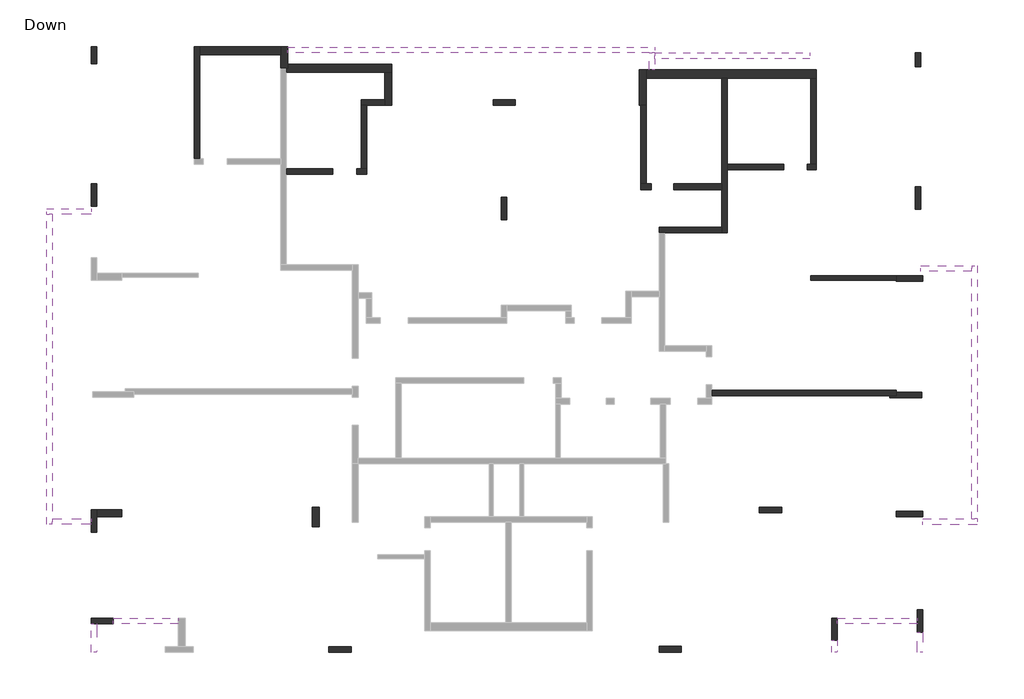
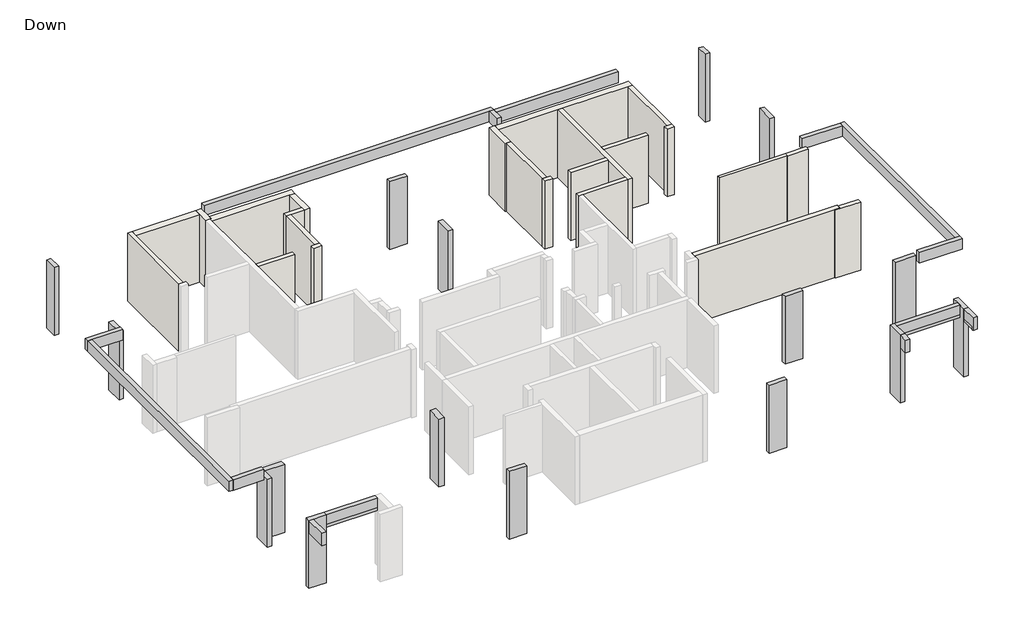
# One storey, part 2 of 2: 23 walls, 16 columns, 14 beams.
"""IFC4 building model written with IfcOpenShell, lengths in millimetres."""

from ifc_helpers import new_model, si_unit, origin, place, context, project, spatial, faceted_brep, element, save

model = new_model("IFC4")

# Units and contexts
model_context = context("Model", 3, world=origin())
ifc_project = project(units=[si_unit("LENGTHUNIT", "METRE", prefix="MILLI")], contexts=[model_context])

# Site, building, storey
site = spatial("IfcSite", under=ifc_project)
building = spatial("IfcBuilding", under=site)
storey = spatial("IfcBuildingStorey", under=building, Name="Down", Elevation=0.0)

# Beams
placement = place(None, origin())
element("IfcBeam", 1, ObjectType="Concrete Rectengular Beam : 20/50", at=placement, inside=storey, context=model_context, shape_type="Brep", body=[
    faceted_brep([(-24231.4241546, 32724.6697375, 3070.0), (-24231.4241546, 32924.6697375, 3070.0), (-24231.4241546, 32924.6697375, 3270.0), (-24231.4241546, 32924.6697375, 3570.0), (-24231.4241546, 32724.6697375, 3570.0), (-24231.4241546, 32724.6697375, 3270.0), (-25831.5472348, 32924.6697375, 3570.0), (-25831.5472348, 32724.6697375, 3570.0), (-25631.5472348, 32724.6697375, 3570.0), (-25831.5472348, 32924.6697375, 3070.0), (-25631.5472348, 32724.6697375, 3070.0), (-25831.5472348, 32724.6697375, 3070.0)], [[[0, 1, 2, 3, 4, 5]], [[4, 3, 6, 7, 8]], [[6, 3, 2, 1, 9]], [[1, 0, 10, 11, 9]], [[4, 8, 7, 11, 10, 0, 5]], [[7, 6, 9, 11]]]),
])
element("IfcBeam", 2, ObjectType="Concrete Rectengular Beam : 20/50", at=placement, inside=storey, context=model_context, shape_type="Brep", body=[
    faceted_brep([(-25831.5472348, 21596.8353122, 3570.0), (-25631.5472348, 21596.8353122, 3570.0), (-25631.5472348, 21796.8353122, 3570.0), (-25631.5472348, 32724.6697375, 3570.0), (-25831.5472348, 32724.6697375, 3570.0), (-25831.5472348, 21596.8353122, 3070.0), (-25831.5472348, 32724.6697375, 3070.0), (-25631.5472348, 21596.8353122, 3070.0), (-25631.5472348, 32724.6697375, 3070.0), (-25631.5472348, 26152.7259194, 3070.0), (-25631.5472348, 21796.8353122, 3070.0), (-25631.5472348, 32724.6697375, 3270.0)], [[[0, 1, 2, 3, 4]], [[5, 0, 4, 6]], [[7, 5, 6, 8, 9, 10]], [[1, 7, 10, 9, 8, 11, 3, 2]], [[1, 0, 5, 7]], [[4, 3, 11, 8, 6]]]),
])
element("IfcBeam", 3, ObjectType="Concrete Rectengular Beam : 20/50", at=placement, inside=storey, context=model_context, shape_type="Brep", body=[
    faceted_brep([(-24232.496199, 21796.8353122, 3570.0), (-24232.496199, 21596.8353122, 3570.0), (-24232.496199, 21596.8353122, 3070.0), (-24232.496199, 21796.8353122, 3070.0), (-24232.496199, 21796.8353122, 3270.0), (-25631.5472348, 21796.8353122, 3570.0), (-25631.5472348, 21596.8353122, 3570.0), (-25631.5472348, 21596.8353122, 3070.0), (-25631.5472348, 21796.8353122, 3070.0), (-25631.5472348, 21796.8353122, 3270.0)], [[[0, 1, 2, 3, 4]], [[1, 0, 5, 6]], [[2, 1, 6, 7]], [[3, 2, 7, 8]], [[4, 3, 8, 9, 5, 0]], [[6, 5, 9, 8, 7]]]),
])
element("IfcBeam", 4, ObjectType="Concrete Rectengular Beam : 20/50", at=placement, inside=storey, context=model_context, shape_type="Brep", body=[
    faceted_brep([(5620.732608, 21792.2762684, 3070.0), (5620.732608, 21592.2762684, 3070.0), (5620.732608, 21592.2762684, 3270.0), (5620.732608, 21592.2762684, 3570.0), (5620.732608, 21792.2762684, 3570.0), (5620.732608, 21792.2762684, 3270.0), (7576.2745907, 21592.2762684, 3570.0), (7576.2745907, 21792.2762684, 3570.0), (7376.2745907, 21792.2762684, 3570.0), (7576.2745907, 21592.2762684, 3070.0), (7376.2745907, 21792.2762684, 3070.0), (7576.2745907, 21792.2762684, 3070.0)], [[[0, 1, 2, 3, 4, 5]], [[4, 3, 6, 7, 8]], [[6, 3, 2, 1, 9]], [[1, 0, 10, 11, 9]], [[4, 8, 7, 11, 10, 0, 5]], [[7, 6, 9, 11]]]),
])
element("IfcBeam", 5, ObjectType="Concrete Rectengular Beam : 20/50", at=placement, inside=storey, context=model_context, shape_type="Brep", body=[
    faceted_brep([(7576.2745907, 30886.4079799, 3570.0), (7376.2745907, 30886.4079799, 3570.0), (7376.2745907, 30686.4079799, 3570.0), (7376.2745907, 21792.2762684, 3570.0), (7576.2745907, 21792.2762684, 3570.0), (7576.2745907, 30886.4079799, 3070.0), (7576.2745907, 21792.2762684, 3070.0), (7376.2745907, 30886.4079799, 3070.0), (7376.2745907, 21792.2762684, 3070.0), (7376.2745907, 26346.3859634, 3070.0), (7376.2745907, 30686.4079799, 3070.0), (7376.2745907, 21792.2762684, 3270.0)], [[[0, 1, 2, 3, 4]], [[5, 0, 4, 6]], [[7, 5, 6, 8, 9, 10]], [[1, 7, 10, 9, 8, 11, 3, 2]], [[4, 3, 11, 8, 6]], [[1, 0, 5, 7]]]),
])
element("IfcBeam", 6, ObjectType="Concrete Rectengular Beam : 20/50", at=placement, inside=storey, context=model_context, shape_type="Brep", body=[
    faceted_brep([(5547.5722379, 30686.4079799, 3570.0), (5547.5722379, 30886.4079799, 3570.0), (5547.5722379, 30886.4079799, 3070.0), (5547.5722379, 30686.4079799, 3070.0), (5547.5722379, 30686.4079799, 3270.0), (7376.2745907, 30686.4079799, 3570.0), (7376.2745907, 30886.4079799, 3570.0), (7376.2745907, 30886.4079799, 3070.0), (7376.2745907, 30686.4079799, 3070.0), (7376.2745907, 30686.4079799, 3270.0)], [[[0, 1, 2, 3, 4]], [[1, 0, 5, 6]], [[2, 1, 6, 7]], [[3, 2, 7, 8]], [[3, 8, 9, 5, 0, 4]], [[7, 6, 5, 9, 8]]]),
])
element("IfcBeam", 7, ObjectType="Concrete Rectengular Beam : 20/50", at=placement, inside=storey, context=model_context, shape_type="Brep", body=[
    faceted_brep([(-17181.9731082, 38714.5374263, 3570.0), (-17181.9731082, 38714.5374263, 3070.0), (-17181.9731082, 38514.5374263, 3070.0), (-17181.9731082, 38514.5374263, 3270.0), (-17181.9731082, 38514.5374263, 3570.0), (-4202.3443382, 38514.5374263, 3570.0), (-4002.3443382, 38514.5374263, 3570.0), (-4002.3443382, 38515.575292, 3570.0), (-4002.3443382, 38714.5374263, 3570.0), (-13700.7193614, 38514.5374263, 3070.0), (-4202.3443382, 38514.5374263, 3070.0), (-4002.3443382, 38514.5374263, 3070.0), (-4002.3443382, 38714.5374263, 3070.0), (-4002.3443382, 38515.575292, 3070.0)], [[[0, 1, 2, 3, 4]], [[0, 4, 5, 6, 7, 8]], [[4, 3, 2, 9, 10, 11, 6, 5]], [[2, 1, 12, 13, 11, 10, 9]], [[1, 0, 8, 12]], [[8, 7, 6, 11, 13, 12]]]),
])
element("IfcBeam", 8, ObjectType="Concrete Rectengular Beam : 20/52", at=placement, inside=storey, context=model_context, shape_type="Brep", body=[
    faceted_brep([(-4002.3443382, 37914.469069, 3570.0), (-4202.3443382, 37914.469069, 3570.0), (-4202.3443382, 37914.469069, 3270.0), (-4202.3443382, 37914.469069, 3070.0), (-4202.3443382, 37914.469069, 3050.0), (-4002.3443382, 37914.469069, 3050.0), (-4002.3443382, 37914.469069, 3070.0), (-4002.3443382, 37914.469069, 3220.0), (-4002.3443382, 38315.575292, 3570.0), (-4002.3443382, 38514.5374263, 3570.0), (-4202.3443382, 38514.5374263, 3570.0), (-4202.3443382, 38515.575292, 3050.0), (-4202.3443382, 38514.5374263, 3270.0), (-4202.3443382, 38514.5374263, 3070.0), (-4202.3443382, 38515.575292, 3070.0), (-4002.3443382, 38515.575292, 3050.0), (-4002.3443382, 38315.575292, 3050.0), (-4002.3443382, 38515.575292, 3070.0), (-4002.3443382, 38514.5374263, 3070.0)], [[[0, 1, 2, 3, 4, 5, 6, 7]], [[1, 0, 8, 9, 10]], [[11, 4, 3, 2, 1, 10, 12, 13, 14]], [[5, 4, 11, 15, 16]], [[0, 7, 6, 5, 16, 15, 17, 18, 9, 8]], [[15, 11, 14, 17]], [[18, 13, 12, 10, 9]], [[13, 18, 17, 14]]]),
])
element("IfcBeam", 9, ObjectType="Concrete Rectengular Beam : 20/52", at=placement, inside=storey, context=model_context, shape_type="Brep", body=[
    faceted_brep([(1566.3525769, 38515.575292, 3570.0), (1566.3525769, 38315.575292, 3570.0), (1566.3525769, 38315.575292, 3270.0), (1566.3525769, 38315.575292, 3070.0), (1566.3525769, 38315.575292, 3050.0), (1566.3525769, 38515.575292, 3050.0), (1566.3525769, 38515.575292, 3070.0), (1566.3525769, 38515.575292, 3270.0), (-4002.3443382, 38515.575292, 3570.0), (-4002.3443382, 38514.5374263, 3570.0), (-4002.3443382, 38315.575292, 3570.0), (-4002.3443382, 38315.575292, 3050.0), (-4002.3443382, 38515.575292, 3050.0), (-4002.3443382, 38515.575292, 3070.0)], [[[0, 1, 2, 3, 4, 5, 6, 7]], [[1, 0, 8, 9, 10]], [[11, 4, 3, 2, 1, 10]], [[5, 4, 11, 12]], [[5, 12, 13, 8, 0, 7, 6]], [[11, 10, 9, 8, 13, 12]]]),
])
element("IfcBeam", 10, ObjectType="Concrete Rectengular Beam : 20/60", at=placement, inside=storey, context=model_context, shape_type="Brep", body=[
    faceted_brep([(5420.732608, 18035.7075634, 3270.0), (5420.732608, 18235.7075634, 3270.0), (2546.318889, 18235.7075634, 3270.0), (2546.318889, 18035.7075634, 3270.0), (2546.318889, 18235.7075634, 2670.0), (2546.318889, 18235.7075634, 3070.0), (5420.732608, 18235.7075634, 3070.0), (5420.732608, 18235.7075634, 2670.0), (5420.732608, 18040.7075634, 2670.0), (2546.318889, 18040.7075634, 2670.0), (2546.318889, 18035.7075634, 2820.0), (5420.732608, 18035.7075634, 2820.0), (5420.732608, 18040.7075634, 2820.0), (2546.318889, 18040.7075634, 2820.0)], [[[0, 1, 2, 3]], [[4, 5, 2, 1, 6, 7]], [[4, 7, 8, 9]], [[0, 3, 10, 11]], [[1, 0, 11, 12, 8, 7, 6]], [[3, 2, 5, 4, 9, 13, 10]], [[13, 12, 11, 10]], [[12, 13, 9, 8]]]),
])
element("IfcBeam", 11, ObjectType="Concrete Rectengular Beam : 20/60", at=placement, inside=storey, context=model_context, shape_type="Brep", body=[
    faceted_brep([(2546.318889, 17016.7180677, 3270.0), (2346.318889, 17016.7180677, 3270.0), (2346.318889, 17016.7180677, 3070.0), (2346.318889, 17016.7180677, 2670.0), (2546.318889, 17016.7180677, 2670.0), (2546.318889, 17435.7075634, 3270.0), (2346.318889, 17435.7075634, 3270.0), (2346.318889, 17435.7075634, 3070.0), (2346.318889, 17435.7075634, 2670.0), (2541.318889, 17435.7075634, 2670.0), (2541.318889, 17066.3078446, 2670.0), (2546.318889, 17066.3078446, 2670.0), (2546.318889, 17066.3078446, 2820.0), (2546.318889, 17435.7075634, 2820.0), (2541.318889, 17435.7075634, 2820.0), (2541.318889, 17066.3078446, 2820.0)], [[[0, 1, 2, 3, 4]], [[1, 0, 5, 6]], [[1, 6, 7, 8, 3, 2]], [[4, 3, 8, 9, 10, 11]], [[0, 4, 11, 12, 13, 5]], [[6, 5, 13, 14, 9, 8, 7]], [[12, 15, 14, 13]], [[10, 15, 12, 11]], [[15, 10, 9, 14]]]),
])
element("IfcBeam", 12, ObjectType="Concrete Rectengular Beam : 20/60", at=placement, inside=storey, context=model_context, shape_type="Brep", body=[
    faceted_brep([(5620.732608, 17010.2006534, 3270.0), (5420.732608, 17010.2006534, 3270.0), (5420.732608, 17010.2006534, 2670.0), (5620.732608, 17010.2006534, 2670.0), (5620.732608, 17735.2006534, 3270.0), (5420.732608, 17735.2006534, 3270.0), (5420.732608, 17735.2006534, 2820.0), (5420.732608, 17066.3078446, 2820.0), (5420.732608, 17066.3078446, 2670.0), (5430.732608, 17066.3078446, 2670.0), (5430.732608, 17735.2006534, 2670.0), (5620.732608, 17735.2006534, 2670.0), (5430.732608, 17735.2006534, 2820.0), (5430.732608, 17066.3078446, 2820.0)], [[[0, 1, 2, 3]], [[1, 0, 4, 5]], [[2, 1, 5, 6, 7, 8]], [[3, 2, 8, 9, 10, 11]], [[0, 3, 11, 4]], [[5, 4, 11, 10, 12, 6]], [[13, 7, 6, 12]], [[13, 9, 8, 7]], [[9, 13, 12, 10]]]),
])
element("IfcBeam", 13, ObjectType="Concrete Rectengular Beam : 20/60", at=placement, inside=storey, context=model_context, shape_type="Brep", body=[
    faceted_brep([(-23432.496199, 18236.7796078, 3270.0), (-23432.496199, 18036.7796078, 3270.0), (-21102.3452666, 18036.7796078, 3270.0), (-21102.3452666, 18236.7796078, 3270.0), (-23432.496199, 18036.7796078, 2820.0), (-21102.3452666, 18036.7796078, 2820.0), (-23432.496199, 18236.7796078, 2670.0), (-21102.3452666, 18236.7796078, 2670.0), (-21102.3452666, 18038.5478478, 2670.0), (-23432.496199, 18038.5478478, 2670.0), (-21102.3452666, 18236.7796078, 3070.0), (-23432.496199, 18236.7796078, 3070.0), (-23432.496199, 18038.5478478, 2820.0), (-21102.3452666, 18038.5478478, 2820.0)], [[[0, 1, 2, 3]], [[2, 1, 4, 5]], [[6, 7, 8, 9]], [[3, 10, 7, 6, 11, 0]], [[1, 0, 11, 6, 9, 12, 4]], [[3, 2, 5, 13, 8, 7, 10]], [[12, 13, 5, 4]], [[13, 12, 9, 8]]]),
])
element("IfcBeam", 14, ObjectType="Concrete Rectengular Beam : 20/60", at=placement, inside=storey, context=model_context, shape_type="Brep", body=[
    faceted_brep([(-24032.496199, 17016.7796078, 3270.0), (-24232.496199, 17016.7796078, 3270.0), (-24232.496199, 17016.7796078, 2670.0), (-24032.496199, 17016.7796078, 2670.0), (-24032.496199, 18036.7796078, 3270.0), (-24232.496199, 18036.7796078, 3270.0), (-24232.496199, 18036.7796078, 2670.0), (-24034.296226, 18036.7796078, 2670.0), (-24034.296226, 17066.3078446, 2670.0), (-24032.496199, 17066.3078446, 2670.0), (-24032.496199, 17066.3078446, 2820.0), (-24032.496199, 18036.7796078, 2820.0), (-24034.296226, 18036.7796078, 2820.0), (-24034.296226, 17066.3078446, 2820.0)], [[[0, 1, 2, 3]], [[1, 0, 4, 5]], [[2, 1, 5, 6]], [[3, 2, 6, 7, 8, 9]], [[0, 3, 9, 10, 11, 4]], [[5, 4, 11, 12, 7, 6]], [[10, 13, 12, 11]], [[8, 13, 10, 9]], [[13, 8, 7, 12]]]),
])

# Columns
element("IfcColumn", 15, ObjectType="Concrete Rectengular Column : 20/50", at=placement, inside=storey, context=model_context, shape_type="Brep", body=[
    faceted_brep([(5346.4978686, 38016.0787934, 0.0), (5346.4978686, 38516.0787934, 0.0), (5546.4978686, 38516.0787934, 0.0), (5546.4978686, 38016.0787934, 0.0), (5346.4978686, 38016.0787934, 3270.0), (5346.4978686, 38515.575292, 3270.0), (5346.4978686, 38516.0787934, 3270.0), (5346.4978686, 38016.0787934, 3070.0), (5546.4978686, 38516.0787934, 3270.0), (5546.4978686, 38016.0787934, 3270.0), (5546.4978686, 38016.0787934, 3070.0)], [[[0, 1, 2, 3]], [[4, 5, 6, 1, 0, 7]], [[6, 8, 2, 1]], [[8, 9, 10, 3, 2]], [[9, 4, 7, 0, 3, 10]], [[4, 9, 8, 6, 5]]]),
])
element("IfcColumn", 16, ObjectType="Concrete Rectengular Column : 20/60", at=placement, inside=storey, context=model_context, shape_type="Brep", body=[
    faceted_brep([(-24231.4241546, 38134.5950671, 0.0), (-24231.4241546, 38734.5950671, 0.0), (-24031.4241546, 38734.5950671, 0.0), (-24031.4241546, 38134.5950671, 0.0), (-24231.4241546, 38134.5950671, 3270.0), (-24231.4241546, 38734.5950671, 3270.0), (-24231.4241546, 38134.5950671, 3070.0), (-24031.4241546, 38734.5950671, 3270.0), (-24031.4241546, 38734.5950671, 3070.0), (-24031.4241546, 38134.5950671, 3270.0), (-24031.4241546, 38134.5950671, 3070.0)], [[[0, 1, 2, 3]], [[4, 5, 1, 0, 6]], [[5, 7, 8, 2, 1]], [[7, 9, 10, 3, 2, 8]], [[9, 4, 6, 0, 3, 10]], [[4, 9, 7, 5]]]),
])
element("IfcColumn", 17, ObjectType="Concrete Rectengular Column : 20/80", at=placement, inside=storey, context=model_context, shape_type="Brep", body=[
    faceted_brep([(-24031.4241546, 33814.6990486, 0.0), (-24031.4241546, 33014.6990486, 0.0), (-24231.4241546, 33014.6990486, 0.0), (-24231.4241546, 33814.6990486, 0.0), (-24031.4241546, 33814.6990486, 3270.0), (-24031.4241546, 33014.6990486, 3270.0), (-24031.4241546, 33014.6990486, 3070.0), (-24031.4241546, 33814.6990486, 3070.0), (-24231.4241546, 33014.6990486, 3270.0), (-24231.4241546, 33014.6990486, 3070.0), (-24231.4241546, 33814.6990486, 3270.0), (-24231.4241546, 33814.6990486, 3070.0)], [[[0, 1, 2, 3]], [[4, 5, 6, 1, 0, 7]], [[5, 8, 9, 2, 1, 6]], [[8, 10, 11, 3, 2, 9]], [[10, 4, 7, 0, 3, 11]], [[4, 10, 8, 5]]]),
])
element("IfcColumn", 18, ObjectType="Concrete Rectengular Column : 20/80", at=placement, inside=storey, context=model_context, shape_type="Brep", body=[
    faceted_brep([(5620.732608, 18535.2006534, 0.0), (5620.732608, 17735.2006534, 0.0), (5420.732608, 17735.2006534, 0.0), (5420.732608, 18535.2006534, 0.0), (5620.732608, 18535.2006534, 3270.0), (5620.732608, 17735.2006534, 3270.0), (5620.732608, 18535.2006534, 3070.0), (5420.732608, 17735.2006534, 3270.0), (5420.732608, 17735.2006534, 2820.0), (5420.732608, 17735.2006534, 2670.0), (5420.732608, 18235.7075634, 3270.0), (5420.732608, 18535.2006534, 3270.0), (5420.732608, 18535.2006534, 3070.0)], [[[0, 1, 2, 3]], [[4, 5, 1, 0, 6]], [[5, 7, 8, 9, 2, 1]], [[7, 10, 11, 12, 3, 2, 9, 8]], [[11, 4, 6, 0, 3, 12]], [[4, 11, 10, 7, 5]]]),
])
element("IfcColumn", 19, ObjectType="Concrete Rectengular Column : 20/80", at=placement, inside=storey, context=model_context, shape_type="Brep", body=[
    faceted_brep([(2546.318889, 18235.7075634, 0.0), (2546.318889, 17435.7075634, 0.0), (2346.318889, 17435.7075634, 0.0), (2346.318889, 18235.7075634, 0.0), (2546.318889, 18235.7075634, 3270.0), (2546.318889, 17435.7075634, 3270.0), (2546.318889, 17435.7075634, 2820.0), (2546.318889, 17435.7075634, 2670.0), (2346.318889, 17435.7075634, 3270.0), (2346.318889, 18235.7075634, 3270.0), (2346.318889, 18235.7075634, 3070.0)], [[[0, 1, 2, 3]], [[4, 5, 6, 7, 1, 0]], [[5, 8, 2, 1, 7, 6]], [[8, 9, 10, 3, 2]], [[9, 4, 0, 3, 10]], [[4, 9, 8, 5]]]),
])
element("IfcColumn", 20, ObjectType="Concrete Rectengular Column : 20/80", at=placement, inside=storey, context=model_context, shape_type="Brep", body=[
    faceted_brep([(-253.8349613, 22214.8479916, 0.0), (546.1650387, 22214.8479916, 0.0), (546.1650387, 22014.8479916, 0.0), (-253.8349613, 22014.8479916, 0.0), (-253.8349613, 22214.8479916, 3270.0), (546.1650387, 22214.8479916, 3270.0), (546.1650387, 22214.8479916, 3070.0), (-253.8349613, 22214.8479916, 3070.0), (546.1650387, 22014.8479916, 3270.0), (546.1650387, 22014.8479916, 3070.0), (-253.8349613, 22014.8479916, 3270.0), (-253.8349613, 22014.8479916, 3070.0)], [[[0, 1, 2, 3]], [[4, 5, 6, 1, 0, 7]], [[5, 8, 9, 2, 1, 6]], [[8, 10, 11, 3, 2, 9]], [[10, 4, 7, 0, 3, 11]], [[4, 10, 8, 5]]]),
])
element("IfcColumn", 21, ObjectType="Concrete Rectengular Column : 20/80", at=placement, inside=storey, context=model_context, shape_type="Brep", body=[
    faceted_brep([(-15702.7330753, 17215.5200253, 0.0), (-14902.7330753, 17215.5200253, 0.0), (-14902.7330753, 17015.5200253, 0.0), (-15702.7330753, 17015.5200253, 0.0), (-15702.7330753, 17215.5200253, 3270.0), (-14902.7330753, 17215.5200253, 3270.0), (-14902.7330753, 17215.5200253, 3070.0), (-15702.7330753, 17215.5200253, 3070.0), (-14902.7330753, 17015.5200253, 3270.0), (-14902.7330753, 17015.5200253, 3070.0), (-15702.7330753, 17015.5200253, 3270.0), (-15702.7330753, 17015.5200253, 3070.0)], [[[0, 1, 2, 3]], [[4, 5, 6, 1, 0, 7]], [[5, 8, 9, 2, 1, 6]], [[8, 10, 11, 3, 2, 9]], [[10, 4, 7, 0, 3, 11]], [[4, 10, 8, 5]]]),
])
element("IfcColumn", 22, ObjectType="Concrete Rectengular Column : 20/80", at=placement, inside=storey, context=model_context, shape_type="Brep", body=[
    faceted_brep([(-24232.496199, 18236.7796078, 0.0), (-23432.496199, 18236.7796078, 0.0), (-23432.496199, 18036.7796078, 0.0), (-24232.496199, 18036.7796078, 0.0), (-24232.496199, 18236.7796078, 3270.0), (-23432.496199, 18236.7796078, 3270.0), (-24232.496199, 18236.7796078, 3070.0), (-23432.496199, 18036.7796078, 3270.0), (-23432.496199, 18036.7796078, 2820.0), (-23432.496199, 18036.7796078, 2670.0), (-24232.496199, 18036.7796078, 3270.0)], [[[0, 1, 2, 3]], [[4, 5, 1, 0, 6]], [[5, 7, 8, 9, 2, 1]], [[7, 10, 3, 2, 9, 8]], [[10, 4, 6, 0, 3]], [[4, 10, 7, 5]]]),
])
element("IfcColumn", 23, ObjectType="Concrete Rectengular Column : 20/80", at=placement, inside=storey, context=model_context, shape_type="Brep", body=[
    faceted_brep([(-24032.496199, 22116.4236302, 0.0), (-24032.496199, 21866.6770852, 0.0), (-24032.496199, 21316.4236302, 0.0), (-24232.496199, 21316.4236302, 0.0), (-24232.496199, 22116.4236302, 0.0), (-24032.496199, 22116.4236302, 3270.0), (-24032.496199, 21866.6770852, 3270.0), (-24032.496199, 21316.4236302, 3270.0), (-24032.496199, 21316.4236302, 3070.0), (-24232.496199, 21316.4236302, 3270.0), (-24232.496199, 21316.4236302, 3070.0), (-24232.496199, 21796.8353122, 3270.0), (-24232.496199, 22116.4236302, 3270.0)], [[[0, 1, 2, 3, 4]], [[5, 6, 7, 8, 2, 1, 0]], [[7, 9, 10, 3, 2, 8]], [[9, 11, 12, 4, 3, 10]], [[12, 5, 0, 4]], [[5, 12, 11, 9, 7, 6]]]),
])
element("IfcColumn", 24, ObjectType="Concrete Rectengular Column : 20/80", at=placement, inside=storey, context=model_context, shape_type="Brep", body=[
    faceted_brep([(5546.4978686, 33715.2026429, 0.0), (5546.4978686, 32915.2026429, 0.0), (5346.4978686, 32915.2026429, 0.0), (5346.4978686, 33715.2026429, 0.0), (5546.4978686, 33715.2026429, 3270.0), (5546.4978686, 32915.2026429, 3270.0), (5546.4978686, 32915.2026429, 3070.0), (5546.4978686, 33715.2026429, 3070.0), (5346.4978686, 32915.2026429, 3270.0), (5346.4978686, 32915.2026429, 3070.0), (5346.4978686, 33715.2026429, 3270.0), (5346.4978686, 33715.2026429, 3070.0)], [[[0, 1, 2, 3]], [[4, 5, 6, 1, 0, 7]], [[5, 8, 9, 2, 1, 6]], [[8, 10, 11, 3, 2, 9]], [[10, 4, 7, 0, 3, 11]], [[4, 10, 8, 5]]]),
])
element("IfcColumn", 25, ObjectType="Concrete Rectengular Column : 20/80", at=placement, inside=storey, context=model_context, shape_type="Brep", body=[
    faceted_brep([(-9808.1078863, 36835.040437, 0.0), (-9008.1078863, 36835.040437, 0.0), (-9008.1078863, 36635.040437, 0.0), (-9808.1078863, 36635.040437, 0.0), (-9808.1078863, 36835.040437, 3270.0), (-9008.1078863, 36835.040437, 3270.0), (-9008.1078863, 36835.040437, 3070.0), (-9808.1078863, 36835.040437, 3070.0), (-9008.1078863, 36635.040437, 3270.0), (-9008.1078863, 36635.040437, 3070.0), (-9808.1078863, 36635.040437, 3270.0), (-9808.1078863, 36635.040437, 3070.0)], [[[0, 1, 2, 3]], [[4, 5, 6, 1, 0, 7]], [[5, 8, 9, 2, 1, 6]], [[8, 10, 11, 3, 2, 9]], [[10, 4, 7, 0, 3, 11]], [[4, 10, 8, 5]]]),
])
element("IfcColumn", 26, ObjectType="Concrete Rectengular Column : 20/80", at=placement, inside=storey, context=model_context, shape_type="Brep", body=[
    faceted_brep([(-9307.5394362, 33336.3391452, 0.0), (-9307.5394362, 32536.3391452, 0.0), (-9507.5394362, 32536.3391452, 0.0), (-9507.5394362, 33336.3391452, 0.0), (-9307.5394362, 33336.3391452, 3270.0), (-9307.5394362, 32536.3391452, 3270.0), (-9307.5394362, 32536.3391452, 3070.0), (-9307.5394362, 33336.3391452, 3070.0), (-9507.5394362, 32536.3391452, 3270.0), (-9507.5394362, 32536.3391452, 3070.0), (-9507.5394362, 33336.3391452, 3270.0), (-9507.5394362, 33336.3391452, 3070.0)], [[[0, 1, 2, 3]], [[4, 5, 6, 1, 0, 7]], [[5, 8, 9, 2, 1, 6]], [[8, 10, 11, 3, 2, 9]], [[10, 4, 7, 0, 3, 11]], [[4, 10, 8, 5]]]),
])
element("IfcColumn", 27, ObjectType="Concrete Rectengular Column : 20/80", at=placement, inside=storey, context=model_context, shape_type="Brep", body=[
    faceted_brep([(-3852.0326588, 17216.7180677, 0.0), (-3052.0326588, 17216.7180677, 0.0), (-3052.0326588, 17016.7180677, 0.0), (-3852.0326588, 17016.7180677, 0.0), (-3852.0326588, 17216.7180677, 3270.0), (-3052.0326588, 17216.7180677, 3270.0), (-3052.0326588, 17216.7180677, 3070.0), (-3852.0326588, 17216.7180677, 3070.0), (-3052.0326588, 17016.7180677, 3270.0), (-3052.0326588, 17016.7180677, 3070.0), (-3852.0326588, 17016.7180677, 3270.0), (-3852.0326588, 17016.7180677, 3070.0)], [[[0, 1, 2, 3]], [[4, 5, 6, 1, 0, 7]], [[5, 8, 9, 2, 1, 6]], [[8, 10, 11, 3, 2, 9]], [[10, 4, 7, 0, 3, 11]], [[4, 10, 8, 5]]]),
])
element("IfcColumn", 28, ObjectType="Concrete Rectengular Column : 20/95", at=placement, inside=storey, context=model_context, shape_type="Brep", body=[
    faceted_brep([(4670.6978259, 22063.1650407, 0.0), (5620.6978259, 22063.1650407, 0.0), (5620.6978259, 21863.1650407, 0.0), (4670.6978259, 21863.1650407, 0.0), (4670.6978259, 22063.1650407, 3270.0), (5620.6978259, 22063.1650407, 3270.0), (5620.6978259, 22063.1650407, 3070.0), (4670.6978259, 22063.1650407, 3070.0), (5620.6978259, 21863.1650407, 3270.0), (5620.6978259, 21863.1650407, 3070.0), (4670.6978259, 21863.1650407, 3270.0), (4670.6978259, 21863.1650407, 3070.0)], [[[0, 1, 2, 3]], [[4, 5, 6, 1, 0, 7]], [[5, 8, 9, 2, 1, 6]], [[8, 10, 11, 3, 2, 9]], [[10, 4, 7, 0, 3, 11]], [[4, 10, 8, 5]]]),
])
element("IfcColumn", 29, ObjectType="Concrete Rectengular Column : 25/110", at=placement, inside=storey, context=model_context, shape_type="Brep", body=[
    faceted_brep([(-24232.496199, 22116.6770852, 0.0), (-23132.496199, 22116.6770852, 0.0), (-23132.496199, 21866.6770852, 0.0), (-24032.496199, 21866.6770852, 0.0), (-24032.496199, 22116.4236302, 0.0), (-24232.496199, 22116.4236302, 0.0), (-24232.496199, 22116.6770852, 3070.0), (-24232.496199, 22116.6770852, 3270.0), (-23132.496199, 22116.6770852, 3270.0), (-23132.496199, 22116.6770852, 3070.0), (-23132.496199, 21866.6770852, 3270.0), (-23132.496199, 21866.6770852, 3070.0), (-24032.496199, 21866.6770852, 3270.0), (-24032.496199, 21866.6770852, 3070.0), (-24232.496199, 22116.4236302, 3270.0), (-24032.496199, 22116.4236302, 3270.0)], [[[0, 1, 2, 3, 4, 5]], [[1, 0, 6, 7, 8, 9]], [[2, 1, 9, 8, 10, 11]], [[2, 11, 10, 12, 13, 3]], [[7, 6, 0, 5, 14]], [[8, 7, 14, 15, 12, 10]], [[15, 4, 3, 13, 12]], [[4, 15, 14, 5]]]),
])
element("IfcColumn", 30, ObjectType="Concrete Rectengular Column : 25/70", at=placement, inside=storey, context=model_context, shape_type="Brep", body=[
    faceted_brep([(-16051.976026, 22215.3208158, 0.0), (-16051.976026, 21515.3208158, 0.0), (-16301.976026, 21515.3208158, 0.0), (-16301.976026, 22215.3208158, 0.0), (-16051.976026, 22215.3208158, 3270.0), (-16051.976026, 21515.3208158, 3270.0), (-16051.976026, 21515.3208158, 3070.0), (-16051.976026, 22215.3208158, 3070.0), (-16301.976026, 21515.3208158, 3270.0), (-16301.976026, 21515.3208158, 3070.0), (-16301.976026, 22215.3208158, 3270.0), (-16301.976026, 22215.3208158, 3070.0)], [[[0, 1, 2, 3]], [[4, 5, 6, 1, 0, 7]], [[5, 8, 9, 2, 1, 6]], [[8, 10, 11, 3, 2, 9]], [[10, 4, 7, 0, 3, 11]], [[4, 10, 8, 5]]]),
])

# Walls
element("IfcWall", 31, ObjectType="15", at=placement, inside=storey, context=model_context, shape_type="Brep", body=[
    faceted_brep([(1598.0523567, 30364.7063432, 0.0), (4667.1364173, 30364.7063432, 0.0), (4667.1364173, 30364.7063432, 3070.0), (4667.1364173, 30364.7063432, 3270.0), (1598.0523567, 30364.7063432, 3270.0), (1598.0523567, 30364.7063432, 3070.0), (1598.0523567, 30514.7063432, 0.0), (1598.0523567, 30514.7063432, 3070.0), (1598.0523567, 30514.7063432, 3270.0), (4667.1364173, 30514.7063432, 3270.0), (4667.1364173, 30514.7063432, 0.0)], [[[0, 1, 2, 3, 4, 5]], [[6, 7, 8, 9, 10]], [[1, 0, 6, 10]], [[3, 2, 1, 10, 9]], [[4, 3, 9, 8]], [[0, 5, 4, 8, 7, 6]]]),
])
element("IfcWall", 32, ObjectType="20", at=placement, inside=storey, context=model_context, shape_type="Brep", body=[
    faceted_brep([(-20332.7228628, 34715.264183, 0.0), (-20332.7228628, 38446.295152, 0.0), (-20332.7228628, 38746.295152, 0.0), (-20332.7228628, 38746.295152, 3270.0), (-20332.7228628, 38446.295152, 3270.0), (-20332.7228628, 34715.264183, 3270.0), (-20332.7228628, 34715.264183, 3070.0), (-20532.7228628, 34715.264183, 0.0), (-20532.7228628, 34715.264183, 3270.0), (-20532.7228628, 38734.5950671, 3270.0), (-20532.7228628, 38746.295152, 3270.0), (-20532.7228628, 38746.295152, 0.0)], [[[0, 1, 2, 3, 4, 5, 6]], [[7, 8, 9, 10, 11]], [[2, 1, 0, 7, 11]], [[5, 4, 3, 10, 9, 8]], [[0, 6, 5, 8, 7]], [[3, 2, 11, 10]]]),
])
element("IfcWall", 33, ObjectType="20", at=placement, inside=storey, context=model_context, shape_type="Brep", body=[
    faceted_brep([(-13700.7193614, 36836.0817113, 0.0), (-14532.2613121, 36836.0817113, 0.0), (-14532.2613121, 36836.0817113, 3070.0), (-14532.2613121, 36836.0817113, 3270.0), (-13700.7193614, 36836.0817113, 3270.0), (-13700.7193614, 36836.0817113, 3070.0), (-13700.7193614, 36636.0817113, 0.0), (-13700.7193614, 36636.0817113, 3270.0), (-14332.2613121, 36636.0817113, 3270.0), (-14532.2613121, 36636.0817113, 3270.0), (-14532.2613121, 36636.0817113, 0.0), (-14332.2613121, 36636.0817113, 0.0)], [[[0, 1, 2, 3, 4, 5]], [[6, 7, 8, 9, 10, 11]], [[1, 0, 6, 11, 10]], [[4, 3, 9, 8, 7]], [[0, 5, 4, 7, 6]], [[3, 2, 1, 10, 9]]]),
])
element("IfcWall", 34, ObjectType="20", at=placement, inside=storey, context=model_context, shape_type="Brep", body=[
    faceted_brep([(-14532.2613121, 36636.0817113, 0.0), (-14532.2613121, 34366.055318, 0.0), (-14532.2613121, 34366.055318, 3070.0), (-14532.2613121, 34366.055318, 3270.0), (-14532.2613121, 36636.0817113, 3270.0), (-14332.2613121, 36636.0817113, 0.0), (-14332.2613121, 36636.0817113, 3070.0), (-14332.2613121, 36636.0817113, 3270.0), (-14332.2613121, 34366.055318, 3270.0), (-14332.2613121, 34366.055318, 0.0)], [[[0, 1, 2, 3, 4]], [[5, 6, 7, 8, 9]], [[1, 0, 5, 9]], [[4, 3, 8, 7]], [[0, 4, 7, 6, 5]], [[3, 2, 1, 9, 8]]]),
])
element("IfcWall", 35, ObjectType="20", at=placement, inside=storey, context=model_context, shape_type="Brep", body=[
    faceted_brep([(-14332.2613121, 34366.055318, 0.0), (-14532.2613121, 34366.055318, 0.0), (-14705.8261281, 34366.055318, 0.0), (-14705.8261281, 34366.055318, 3070.0), (-14705.8261281, 34366.055318, 3270.0), (-14532.2613121, 34366.055318, 3270.0), (-14332.2613121, 34366.055318, 3270.0), (-14332.2613121, 34166.055318, 0.0), (-14332.2613121, 34166.055318, 3070.0), (-14332.2613121, 34166.055318, 3270.0), (-14705.8261281, 34166.055318, 3270.0), (-14705.8261281, 34166.055318, 3070.0), (-14705.8261281, 34166.055318, 0.0)], [[[0, 1, 2, 3, 4, 5, 6]], [[7, 8, 9, 10, 11, 12]], [[2, 1, 0, 7, 12]], [[4, 3, 2, 12, 11, 10]], [[6, 5, 4, 10, 9]], [[0, 6, 9, 8, 7]]]),
])
element("IfcWall", 36, ObjectType="20", at=placement, inside=storey, context=model_context, shape_type="Brep", body=[
    faceted_brep([(-15560.9362106, 34366.055318, 0.0), (-17231.9731082, 34366.055318, 0.0), (-17231.9731082, 34366.055318, 3070.0), (-17231.9731082, 34366.055318, 3270.0), (-15560.9362106, 34366.055318, 3270.0), (-15560.9362106, 34366.055318, 3070.0), (-15560.9362106, 34166.055318, 0.0), (-15560.9362106, 34166.055318, 3070.0), (-15560.9362106, 34166.055318, 3270.0), (-17231.9731082, 34166.055318, 3270.0), (-17231.9731082, 34166.055318, 3070.0), (-17231.9731082, 34166.055318, 0.0)], [[[0, 1, 2, 3, 4, 5]], [[6, 7, 8, 9, 10, 11]], [[1, 0, 6, 11]], [[4, 3, 9, 8]], [[0, 5, 4, 8, 7, 6]], [[3, 2, 1, 11, 10, 9]]]),
])
element("IfcWall", 37, ObjectType="20", at=placement, inside=storey, context=model_context, shape_type="Brep", body=[
    faceted_brep([(-4301.8715139, 33815.7403229, 0.0), (-4301.8715139, 36636.0817113, 0.0), (-4301.8715139, 36636.0817113, 3070.0), (-4301.8715139, 36636.0817113, 3270.0), (-4301.8715139, 33815.7403229, 3270.0), (-4301.8715139, 33815.7403229, 3070.0), (-4501.8715139, 33815.7403229, 0.0), (-4501.8715139, 33815.7403229, 3270.0), (-4501.8715139, 36636.0817113, 3270.0), (-4501.8715139, 36636.0817113, 3070.0), (-4501.8715139, 36636.0817113, 0.0), (-4302.6593333, 36636.0817113, 0.0), (-4302.6593333, 36636.0817113, 3270.0)], [[[0, 1, 2, 3, 4, 5]], [[6, 7, 8, 9, 10]], [[1, 0, 6, 10, 11]], [[3, 2, 1, 11, 10, 9, 8, 12]], [[4, 3, 12, 8, 7]], [[0, 5, 4, 7, 6]]]),
])
element("IfcWall", 38, ObjectType="20", at=placement, inside=storey, context=model_context, shape_type="Brep", body=[
    faceted_brep([(-4501.8715139, 33615.7403229, 0.0), (-4138.8749491, 33615.7403229, 0.0), (-4138.8749491, 33615.7403229, 3070.0), (-4138.8749491, 33615.7403229, 3270.0), (-4501.8715139, 33615.7403229, 3270.0), (-4501.8715139, 33615.7403229, 3070.0), (-4501.8715139, 33815.7403229, 0.0), (-4501.8715139, 33815.7403229, 3270.0), (-4301.8715139, 33815.7403229, 3270.0), (-4138.8749491, 33815.7403229, 3270.0), (-4138.8749491, 33815.7403229, 3070.0), (-4138.8749491, 33815.7403229, 0.0), (-4301.8715139, 33815.7403229, 0.0)], [[[0, 1, 2, 3, 4, 5]], [[6, 7, 8, 9, 10, 11, 12]], [[1, 0, 6, 12, 11]], [[3, 2, 1, 11, 10, 9]], [[4, 3, 9, 8, 7]], [[0, 5, 4, 7, 6]]]),
])
element("IfcWall", 39, ObjectType="20", at=placement, inside=storey, context=model_context, shape_type="Brep", body=[
    faceted_brep([(-3320.8331575, 33615.7403229, 0.0), (-1603.2009922, 33615.7403229, 0.0), (-1603.2009922, 33615.7403229, 3070.0), (-1603.2009922, 33615.7403229, 3270.0), (-3320.8331575, 33615.7403229, 3270.0), (-3320.8331575, 33615.7403229, 3070.0), (-3320.8331575, 33815.7403229, 0.0), (-3320.8331575, 33815.7403229, 3070.0), (-3320.8331575, 33815.7403229, 3270.0), (-1603.2009922, 33815.7403229, 3270.0), (-1603.2009922, 33815.7403229, 3070.0), (-1603.2009922, 33815.7403229, 0.0)], [[[0, 1, 2, 3, 4, 5]], [[6, 7, 8, 9, 10, 11]], [[1, 0, 6, 11]], [[4, 3, 9, 8]], [[0, 5, 4, 8, 7, 6]], [[3, 2, 1, 11, 10, 9]]]),
])
element("IfcWall", 40, ObjectType="20", at=placement, inside=storey, context=model_context, shape_type="Brep", body=[
    faceted_brep([(-1603.2009922, 37614.469069, 0.0), (-1603.2009922, 33815.7403229, 0.0), (-1603.2009922, 33615.7403229, 0.0), (-1603.2009922, 32266.405062, 0.0), (-1603.2009922, 32066.405062, 0.0), (-1603.2009922, 32066.405062, 3270.0), (-1603.2009922, 32266.405062, 3270.0), (-1603.2009922, 33615.7403229, 3270.0), (-1603.2009922, 33815.7403229, 3270.0), (-1603.2009922, 37614.469069, 3270.0), (-1603.2009922, 37614.469069, 3070.0), (-1403.2009922, 37614.469069, 0.0), (-1403.2009922, 37614.469069, 3070.0), (-1403.2009922, 37614.469069, 3270.0), (-1403.2009922, 34516.3054573, 3270.0), (-1403.2009922, 34316.3054573, 3270.0), (-1403.2009922, 32066.405062, 3270.0), (-1403.2009922, 32066.405062, 3070.0), (-1403.2009922, 32066.405062, 0.0), (-1403.2009922, 34316.3054573, 0.0), (-1403.2009922, 34516.3054573, 0.0)], [[[0, 1, 2, 3, 4, 5, 6, 7, 8, 9, 10]], [[11, 12, 13, 14, 15, 16, 17, 18, 19, 20]], [[4, 3, 2, 1, 0, 11, 20, 19, 18]], [[9, 8, 7, 6, 5, 16, 15, 14, 13]], [[0, 10, 9, 13, 12, 11]], [[5, 4, 18, 17, 16]]]),
])
element("IfcWall", 41, ObjectType="20", at=placement, inside=storey, context=model_context, shape_type="Brep", body=[
    faceted_brep([(1597.1133398, 37614.469069, 0.0), (1597.1133398, 34516.3054573, 0.0), (1597.1133398, 34516.3054573, 3070.0), (1597.1133398, 34516.3054573, 3270.0), (1597.1133398, 37614.469069, 3270.0), (1597.1133398, 37614.469069, 3070.0), (1797.1133398, 37614.469069, 0.0), (1797.1133398, 37614.469069, 3270.0), (1797.1133398, 34516.3054573, 3270.0), (1797.1133398, 34516.3054573, 0.0)], [[[0, 1, 2, 3, 4, 5]], [[6, 7, 8, 9]], [[1, 0, 6, 9]], [[4, 3, 8, 7]], [[0, 5, 4, 7, 6]], [[3, 2, 1, 9, 8]]]),
])
element("IfcWall", 42, ObjectType="20", at=placement, inside=storey, context=model_context, shape_type="Brep", body=[
    faceted_brep([(1797.1133398, 34516.3054573, 0.0), (1597.1133398, 34516.3054573, 0.0), (1475.3435315, 34516.3054573, 0.0), (1475.3435315, 34516.3054573, 3070.0), (1475.3435315, 34516.3054573, 3270.0), (1597.1133398, 34516.3054573, 3270.0), (1797.1133398, 34516.3054573, 3270.0), (1797.1133398, 34316.3054573, 0.0), (1797.1133398, 34316.3054573, 3070.0), (1797.1133398, 34316.3054573, 3270.0), (1475.3435315, 34316.3054573, 3270.0), (1475.3435315, 34316.3054573, 3070.0), (1475.3435315, 34316.3054573, 0.0)], [[[0, 1, 2, 3, 4, 5, 6]], [[7, 8, 9, 10, 11, 12]], [[2, 1, 0, 7, 12]], [[4, 3, 2, 12, 11, 10]], [[6, 5, 4, 10, 9]], [[0, 6, 9, 8, 7]]]),
])
element("IfcWall", 43, ObjectType="20", at=placement, inside=storey, context=model_context, shape_type="Brep", body=[
    faceted_brep([(620.1311917, 34516.3054573, 0.0), (-1403.2009922, 34516.3054573, 0.0), (-1403.2009922, 34516.3054573, 3070.0), (-1403.2009922, 34516.3054573, 3270.0), (620.1311917, 34516.3054573, 3270.0), (620.1311917, 34516.3054573, 3070.0), (620.1311917, 34316.3054573, 0.0), (620.1311917, 34316.3054573, 3070.0), (620.1311917, 34316.3054573, 3270.0), (-1403.2009922, 34316.3054573, 3270.0), (-1403.2009922, 34316.3054573, 3070.0), (-1403.2009922, 34316.3054573, 0.0)], [[[0, 1, 2, 3, 4, 5]], [[6, 7, 8, 9, 10, 11]], [[1, 0, 6, 11]], [[4, 3, 9, 8]], [[0, 5, 4, 8, 7, 6]], [[3, 2, 1, 11, 10, 9]]]),
])
element("IfcWall", 44, ObjectType="20", at=placement, inside=storey, context=model_context, shape_type="Brep", body=[
    faceted_brep([(-1603.2009922, 32266.405062, 0.0), (-3852.0941989, 32266.405062, 0.0), (-3852.0941989, 32266.405062, 3070.0), (-3852.0941989, 32266.405062, 3270.0), (-1603.2009922, 32266.405062, 3270.0), (-1603.2009922, 32266.405062, 3070.0), (-1603.2009922, 32066.405062, 0.0), (-1603.2009922, 32066.405062, 3270.0), (-3652.0941989, 32066.405062, 3270.0), (-3852.0941989, 32066.405062, 3270.0), (-3852.0941989, 32066.405062, 0.0), (-3652.0941989, 32066.405062, 0.0)], [[[0, 1, 2, 3, 4, 5]], [[6, 7, 8, 9, 10, 11]], [[1, 0, 6, 11, 10]], [[4, 3, 9, 8, 7]], [[0, 5, 4, 7, 6]], [[3, 2, 1, 10, 9]]]),
])
element("IfcWall", 45, ObjectType="20", at=placement, inside=storey, context=model_context, shape_type="Brep", body=[
    faceted_brep([(-1953.6864162, 26215.1864621, 0.0), (4427.8542082, 26215.1864621, 0.0), (4656.569824, 26215.1864621, 0.0), (4656.569824, 26215.1864621, 3270.0), (4427.8542082, 26215.1864621, 3270.0), (-1953.6864162, 26215.1864621, 3270.0), (-1953.6864162, 26215.1864621, 3070.0), (-1953.6864162, 26415.1864621, 0.0), (-1953.6864162, 26415.1864621, 3070.0), (-1953.6864162, 26415.1864621, 3270.0), (4656.569824, 26415.1864621, 3270.0), (4656.569824, 26415.1864621, 3070.0), (4656.569824, 26415.1864621, 0.0), (4656.569824, 26346.3859634, 0.0), (4656.569824, 26346.3859634, 3270.0)], [[[0, 1, 2, 3, 4, 5, 6]], [[7, 8, 9, 10, 11, 12]], [[2, 1, 0, 7, 12, 13]], [[3, 2, 13, 12, 11, 10, 14]], [[5, 4, 3, 14, 10, 9]], [[0, 6, 5, 9, 8, 7]]]),
])
element("IfcWall", 46, ObjectType="20", at=placement, inside=storey, context=model_context, shape_type="Brep", body=[
    faceted_brep([(4427.8542082, 26146.3859634, 0.0), (5577.2268706, 26146.3859634, 0.0), (5577.2268706, 26146.3859634, 3070.0), (5577.2268706, 26146.3859634, 3270.0), (4427.8542082, 26146.3859634, 3270.0), (4427.8542082, 26146.3859634, 3070.0), (5577.2268706, 26346.3859634, 3270.0), (5577.2268706, 26346.3859634, 3070.0), (5577.2268706, 26346.3859634, 0.0), (4656.569824, 26346.3859634, 0.0), (4656.569824, 26346.3859634, 3070.0), (4656.569824, 26346.3859634, 3270.0), (4427.8542082, 26215.1864621, 0.0), (4656.569824, 26215.1864621, 0.0), (4656.569824, 26215.1864621, 3270.0), (4427.8542082, 26215.1864621, 3270.0), (4427.8542082, 26215.1864621, 3070.0)], [[[0, 1, 2, 3, 4, 5]], [[6, 7, 8, 9, 10, 11]], [[1, 0, 12, 13, 9, 8]], [[3, 2, 1, 8, 7, 6]], [[4, 3, 6, 11, 14, 15]], [[0, 5, 4, 15, 16, 12]], [[14, 13, 12, 16, 15]], [[13, 14, 11, 10, 9]]]),
])
element("IfcWall", 47, ObjectType="20", at=placement, inside=storey, context=model_context, shape_type="Brep", body=[
    faceted_brep([(4667.1364173, 30314.7063432, 0.0), (5607.1364173, 30314.7063432, 0.0), (5607.1364173, 30314.7063432, 3070.0), (5607.1364173, 30314.7063432, 3270.0), (4667.1364173, 30314.7063432, 3270.0), (4667.1364173, 30314.7063432, 3070.0), (4667.1364173, 30514.7063432, 0.0), (4667.1364173, 30514.7063432, 3270.0), (5607.1364173, 30514.7063432, 3270.0), (5607.1364173, 30514.7063432, 3070.0), (5607.1364173, 30514.7063432, 0.0), (4667.1364173, 30364.7063432, 0.0), (4667.1364173, 30364.7063432, 3270.0)], [[[0, 1, 2, 3, 4, 5]], [[6, 7, 8, 9, 10]], [[1, 0, 11, 6, 10]], [[3, 2, 1, 10, 9, 8]], [[4, 3, 8, 7, 12]], [[0, 5, 4, 12, 7, 6, 11]]]),
])
element("IfcWall", 48, ObjectType="25", at=placement, inside=storey, context=model_context, shape_type="Brep", body=[
    faceted_brep([(-17431.9731082, 38746.295152, 0.0), (-17431.9731082, 38446.295152, 0.0), (-17431.9731082, 37965.0067491, 0.0), (-17431.9731082, 37965.0067491, 3270.0), (-17431.9731082, 38446.295152, 3270.0), (-17431.9731082, 38746.295152, 3270.0), (-17181.9731082, 38746.295152, 0.0), (-17181.9731082, 38746.295152, 3270.0), (-17181.9731082, 38514.5374263, 3270.0), (-17181.9731082, 38115.0067491, 3270.0), (-17181.9731082, 37965.0067491, 3270.0), (-17181.9731082, 37965.0067491, 0.0), (-17181.9731082, 38115.0067491, 0.0), (-17231.9731082, 37965.0067491, 0.0), (-17231.9731082, 37965.0067491, 3270.0)], [[[0, 1, 2, 3, 4, 5]], [[6, 7, 8, 9, 10, 11, 12]], [[2, 1, 0, 6, 12, 11, 13]], [[3, 2, 13, 11, 10, 14]], [[5, 4, 3, 14, 10, 9, 8, 7]], [[0, 5, 7, 6]]]),
])
element("IfcWall", 49, ObjectType="25", at=placement, inside=storey, context=model_context, shape_type="Brep", body=[
    faceted_brep([(-13700.7193614, 37815.0067491, 0.0), (-13700.7193614, 36836.0817113, 0.0), (-13700.7193614, 36636.0817113, 0.0), (-13700.7193614, 36636.0817113, 3270.0), (-13700.7193614, 36836.0817113, 3270.0), (-13700.7193614, 37815.0067491, 3270.0), (-13700.7193614, 37815.0067491, 3070.0), (-13450.7193614, 37815.0067491, 0.0), (-13450.7193614, 37815.0067491, 3270.0), (-13450.7193614, 36636.0817113, 3270.0), (-13450.7193614, 36636.0817113, 3070.0), (-13450.7193614, 36636.0817113, 0.0)], [[[0, 1, 2, 3, 4, 5, 6]], [[7, 8, 9, 10, 11]], [[2, 1, 0, 7, 11]], [[5, 4, 3, 9, 8]], [[0, 6, 5, 8, 7]], [[3, 2, 11, 10, 9]]]),
])
element("IfcWall", 50, ObjectType="25", at=placement, inside=storey, context=model_context, shape_type="Brep", body=[
    faceted_brep([(-4302.6593333, 36636.0817113, 0.0), (-4302.6593333, 37614.469069, 0.0), (-4302.6593333, 37914.469069, 0.0), (-4302.6593333, 37914.469069, 3270.0), (-4302.6593333, 37614.469069, 3270.0), (-4302.6593333, 36636.0817113, 3270.0), (-4302.6593333, 36636.0817113, 3070.0), (-4552.6593333, 36636.0817113, 0.0), (-4552.6593333, 36636.0817113, 3070.0), (-4552.6593333, 36636.0817113, 3270.0), (-4552.6593333, 37914.469069, 3270.0), (-4552.6593333, 37914.469069, 3070.0), (-4552.6593333, 37914.469069, 0.0), (-4501.8715139, 36636.0817113, 0.0), (-4501.8715139, 36636.0817113, 3270.0)], [[[0, 1, 2, 3, 4, 5, 6]], [[7, 8, 9, 10, 11, 12]], [[2, 1, 0, 13, 7, 12]], [[5, 4, 3, 10, 9, 14]], [[0, 6, 5, 14, 9, 8, 7, 13]], [[3, 2, 12, 11, 10]]]),
])
element("IfcWall", 51, ObjectType="30", at=placement, inside=storey, context=model_context, shape_type="Brep", body=[
    faceted_brep([(-20332.7228628, 38446.295152, 0.0), (-17431.9731082, 38446.295152, 0.0), (-17431.9731082, 38446.295152, 3070.0), (-17431.9731082, 38446.295152, 3270.0), (-20332.7228628, 38446.295152, 3270.0), (-20332.7228628, 38446.295152, 3070.0), (-20332.7228628, 38746.295152, 0.0), (-20332.7228628, 38746.295152, 3270.0), (-17431.9731082, 38746.295152, 3270.0), (-17431.9731082, 38746.295152, 0.0)], [[[0, 1, 2, 3, 4, 5]], [[6, 7, 8, 9]], [[1, 0, 6, 9]], [[4, 3, 8, 7]], [[0, 5, 4, 7, 6]], [[3, 2, 1, 9, 8]]]),
])
element("IfcWall", 52, ObjectType="30", at=placement, inside=storey, context=model_context, shape_type="Brep", body=[
    faceted_brep([(-17231.9731082, 37815.0067491, 0.0), (-13700.7193614, 37815.0067491, 0.0), (-13450.7193614, 37815.0067491, 0.0), (-13450.7193614, 37815.0067491, 3270.0), (-13700.7193614, 37815.0067491, 3270.0), (-17231.9731082, 37815.0067491, 3270.0), (-17231.9731082, 37815.0067491, 3070.0), (-17181.9731082, 38115.0067491, 0.0), (-17181.9731082, 38115.0067491, 3070.0), (-17181.9731082, 38115.0067491, 3270.0), (-13700.7193614, 38115.0067491, 3270.0), (-13450.7193614, 38115.0067491, 3270.0), (-13450.7193614, 38115.0067491, 3070.0), (-13450.7193614, 38115.0067491, 0.0), (-17231.9731082, 37965.0067491, 0.0), (-17181.9731082, 37965.0067491, 0.0), (-17181.9731082, 37965.0067491, 3270.0), (-17231.9731082, 37965.0067491, 3270.0)], [[[0, 1, 2, 3, 4, 5, 6]], [[7, 8, 9, 10, 11, 12, 13]], [[2, 1, 0, 14, 15, 7, 13]], [[5, 4, 3, 11, 10, 9, 16, 17]], [[0, 6, 5, 17, 14]], [[17, 16, 15, 14]], [[16, 9, 8, 7, 15]], [[3, 2, 13, 12, 11]]]),
])
element("IfcWall", 53, ObjectType="30", at=placement, inside=storey, context=model_context, shape_type="Brep", body=[
    faceted_brep([(-4302.6593333, 37614.469069, 0.0), (-1603.2009922, 37614.469069, 0.0), (-1403.2009922, 37614.469069, 0.0), (1597.1133398, 37614.469069, 0.0), (1797.1133398, 37614.469069, 0.0), (1797.1133398, 37614.469069, 3270.0), (1597.1133398, 37614.469069, 3270.0), (-1403.2009922, 37614.469069, 3270.0), (-1603.2009922, 37614.469069, 3270.0), (-4302.6593333, 37614.469069, 3270.0), (-4302.6593333, 37614.469069, 3070.0), (-4302.6593333, 37914.469069, 0.0), (-4302.6593333, 37914.469069, 3270.0), (-4202.3443382, 37914.469069, 3270.0), (1566.3525769, 37914.469069, 3270.0), (1797.1133398, 37914.469069, 3270.0), (1797.1133398, 37914.469069, 3070.0), (1797.1133398, 37914.469069, 0.0)], [[[0, 1, 2, 3, 4, 5, 6, 7, 8, 9, 10]], [[11, 12, 13, 14, 15, 16, 17]], [[4, 3, 2, 1, 0, 11, 17]], [[9, 8, 7, 6, 5, 15, 14, 13, 12]], [[0, 10, 9, 12, 11]], [[5, 4, 17, 16, 15]]]),
])

save(model, "model.ifc")

# Revit data of these elements
# Type "Concrete Rectengular Beam : 20/50"
#   Length [instance default] = 152.4 cm
#   b = 20 cm
#   h = 50 cm
#   Structural Material [instance default] = Concrete
#   Assembly Code = ""
# Type "Concrete Rectengular Beam : 20/52"
#   Length [instance default] = 152.4 cm
#   b = 20 cm
#   h = 52 cm
#   Structural Material [instance default] = Concrete
#   Assembly Code = ""
# Type "Concrete Rectengular Beam : 20/60"
#   Length [instance default] = 152.4 cm
#   b = 20 cm
#   h = 60 cm
#   Structural Material [instance default] = Concrete
#   Assembly Code = ""
# Type "Concrete Rectengular Column : 20/50"
#   b = 20 cm
#   h = 50 cm
#   Structural Material [instance default] = Concrete
# Type "Concrete Rectengular Column : 20/60"
#   b = 20 cm
#   h = 60 cm
#   Structural Material [instance default] = Concrete
# Type "Concrete Rectengular Column : 20/80"
#   b = 20 cm
#   h = 80 cm
#   Structural Material [instance default] = Concrete
# Type "Concrete Rectengular Column : 20/95"
#   b = 20 cm
#   h = 95 cm
#   Structural Material [instance default] = Concrete
# Type "Concrete Rectengular Column : 25/110"
#   b = 25 cm
#   h = 110 cm
#   Structural Material [instance default] = Concrete
# Type "Concrete Rectengular Column : 25/70"
#   b = 25 cm
#   h = 70 cm
#   Structural Material [instance default] = Concrete
# Type "15"
#   Layers, outside or top first: 15 cm "Concrete" (function 1)
# Type "20"
#   Layers, outside or top first: 20 cm "Concrete" (function 1)
# Type "25"
#   Layers, outside or top first: 25 cm "Concrete" (function 1)
# Type "30"
#   Layers, outside or top first: 30 cm "Concrete" (function 1)
# Element 1 (IfcBeam, "Concrete Rectengular Beam : 20/50")
#   Comments = ""
#   Mark = "B1"
#   SOFiSTiK_AMG_Comments = ""
#   SOFiSTiK_AMG_Scheduled = yes
#   SOFiSTiK_AMG_Adjusted = yes
#   Structural Material = Concrete
#   Phase Created = New Construction
#   Materials on its faces: "Concrete"
# Element 2 (IfcBeam, "Concrete Rectengular Beam : 20/50")
#   Comments = ""
#   Mark = "B2"
#   SOFiSTiK_AMG_Comments = ""
#   SOFiSTiK_AMG_Scheduled = yes
#   SOFiSTiK_AMG_Adjusted = yes
#   Structural Material = Concrete
#   Phase Created = New Construction
#   Materials on its faces: "Concrete"
# Element 3 (IfcBeam, "Concrete Rectengular Beam : 20/50")
#   Comments = ""
#   Mark = "B3"
#   SOFiSTiK_AMG_Comments = ""
#   SOFiSTiK_AMG_Scheduled = yes
#   SOFiSTiK_AMG_Adjusted = yes
#   Structural Material = Concrete
#   Phase Created = New Construction
#   Materials on its faces: "Concrete"
# Element 4 (IfcBeam, "Concrete Rectengular Beam : 20/50")
#   Comments = ""
#   Mark = "B4"
#   SOFiSTiK_AMG_Comments = ""
#   SOFiSTiK_AMG_Scheduled = yes
#   SOFiSTiK_AMG_Adjusted = yes
#   Structural Material = Concrete
#   Phase Created = New Construction
#   Materials on its faces: "Concrete"
# Element 5 (IfcBeam, "Concrete Rectengular Beam : 20/50")
#   Comments = ""
#   Mark = "B5"
#   SOFiSTiK_AMG_Comments = ""
#   SOFiSTiK_AMG_Scheduled = yes
#   SOFiSTiK_AMG_Adjusted = yes
#   Structural Material = Concrete
#   Phase Created = New Construction
#   Materials on its faces: "Concrete"
# Element 6 (IfcBeam, "Concrete Rectengular Beam : 20/50")
#   Comments = ""
#   Mark = "B6"
#   SOFiSTiK_AMG_Comments = ""
#   SOFiSTiK_AMG_Scheduled = yes
#   SOFiSTiK_AMG_Adjusted = yes
#   Structural Material = Concrete
#   Phase Created = New Construction
#   Materials on its faces: "Concrete"
# Element 7 (IfcBeam, "Concrete Rectengular Beam : 20/50")
#   Comments = ""
#   Mark = "B7"
#   SOFiSTiK_AMG_Comments = ""
#   SOFiSTiK_AMG_Scheduled = yes
#   SOFiSTiK_AMG_Adjusted = yes
#   Structural Material = Concrete
#   Phase Created = New Construction
#   Materials on its faces: "Concrete"
# Element 8 (IfcBeam, "Concrete Rectengular Beam : 20/52")
#   Comments = ""
#   Mark = "B8"
#   SOFiSTiK_AMG_Comments = ""
#   SOFiSTiK_AMG_Scheduled = yes
#   SOFiSTiK_AMG_Adjusted = yes
#   Structural Material = Concrete
#   Phase Created = New Construction
#   Materials on its faces: "Concrete"
# Element 9 (IfcBeam, "Concrete Rectengular Beam : 20/52")
#   Comments = ""
#   Mark = "B9"
#   SOFiSTiK_AMG_Comments = ""
#   SOFiSTiK_AMG_Scheduled = yes
#   SOFiSTiK_AMG_Adjusted = yes
#   Structural Material = Concrete
#   Phase Created = New Construction
#   Materials on its faces: "Concrete"
# Element 10 (IfcBeam, "Concrete Rectengular Beam : 20/60")
#   Comments = ""
#   Mark = "B10"
#   SOFiSTiK_AMG_Comments = ""
#   SOFiSTiK_AMG_Scheduled = yes
#   SOFiSTiK_AMG_Adjusted = yes
#   Structural Material = Concrete
#   Phase Created = New Construction
#   Materials on its faces: "Concrete"
# Element 11 (IfcBeam, "Concrete Rectengular Beam : 20/60")
#   Comments = ""
#   Mark = "B11"
#   SOFiSTiK_AMG_Comments = ""
#   SOFiSTiK_AMG_Scheduled = yes
#   SOFiSTiK_AMG_Adjusted = yes
#   Structural Material = Concrete
#   Phase Created = New Construction
#   Materials on its faces: "Concrete"
# Element 12 (IfcBeam, "Concrete Rectengular Beam : 20/60")
#   Comments = ""
#   Mark = "B12"
#   SOFiSTiK_AMG_Comments = ""
#   SOFiSTiK_AMG_Scheduled = yes
#   SOFiSTiK_AMG_Adjusted = yes
#   Structural Material = Concrete
#   Phase Created = New Construction
#   Materials on its faces: "Concrete"
# Element 13 (IfcBeam, "Concrete Rectengular Beam : 20/60")
#   Comments = ""
#   Mark = "B13"
#   SOFiSTiK_AMG_Comments = ""
#   SOFiSTiK_AMG_Scheduled = yes
#   SOFiSTiK_AMG_Adjusted = yes
#   Structural Material = Concrete
#   Phase Created = New Construction
#   Materials on its faces: "Concrete"
# Element 14 (IfcBeam, "Concrete Rectengular Beam : 20/60")
#   Comments = ""
#   Mark = "B14"
#   SOFiSTiK_AMG_Comments = ""
#   SOFiSTiK_AMG_Scheduled = yes
#   SOFiSTiK_AMG_Adjusted = yes
#   Structural Material = Concrete
#   Phase Created = New Construction
#   Materials on its faces: "Concrete"
# Element 15 (IfcColumn, "Concrete Rectengular Column : 20/50")
#   Comments = ""
#   Mark = "C1"
#   SOFiSTiK_AMG_Comments = ""
#   SOFiSTiK_AMG_Scheduled = yes
#   SOFiSTiK_AMG_Adjusted = yes
#   Structural Material = Concrete
#   Phase Created = New Construction
#   Materials on its faces: "Concrete"
# Element 16 (IfcColumn, "Concrete Rectengular Column : 20/60")
#   Comments = ""
#   Mark = "C2"
#   SOFiSTiK_AMG_Comments = ""
#   SOFiSTiK_AMG_Scheduled = yes
#   SOFiSTiK_AMG_Adjusted = yes
#   Structural Material = Concrete
#   Phase Created = New Construction
#   Materials on its faces: "Concrete"
# Element 17 (IfcColumn, "Concrete Rectengular Column : 20/80")
#   Comments = ""
#   Mark = "C3"
#   SOFiSTiK_AMG_Comments = ""
#   SOFiSTiK_AMG_Scheduled = yes
#   SOFiSTiK_AMG_Adjusted = yes
#   Structural Material = Concrete
#   Phase Created = New Construction
#   Materials on its faces: "Concrete"
# Element 18 (IfcColumn, "Concrete Rectengular Column : 20/80")
#   Comments = ""
#   Mark = "C4"
#   SOFiSTiK_AMG_Comments = ""
#   SOFiSTiK_AMG_Scheduled = yes
#   SOFiSTiK_AMG_Adjusted = yes
#   Structural Material = Concrete
#   Phase Created = New Construction
#   Materials on its faces: "Concrete"
# Element 19 (IfcColumn, "Concrete Rectengular Column : 20/80")
#   Comments = ""
#   Mark = "C5"
#   SOFiSTiK_AMG_Comments = ""
#   SOFiSTiK_AMG_Scheduled = yes
#   SOFiSTiK_AMG_Adjusted = yes
#   Structural Material = Concrete
#   Phase Created = New Construction
#   Materials on its faces: "Concrete"
# Element 20 (IfcColumn, "Concrete Rectengular Column : 20/80")
#   Comments = ""
#   Mark = "C6"
#   SOFiSTiK_AMG_Comments = ""
#   SOFiSTiK_AMG_Scheduled = yes
#   SOFiSTiK_AMG_Adjusted = yes
#   Structural Material = Concrete
#   Phase Created = New Construction
#   Materials on its faces: "Concrete"
# Element 21 (IfcColumn, "Concrete Rectengular Column : 20/80")
#   Comments = ""
#   Mark = "C7"
#   SOFiSTiK_AMG_Comments = ""
#   SOFiSTiK_AMG_Scheduled = yes
#   SOFiSTiK_AMG_Adjusted = yes
#   Structural Material = Concrete
#   Phase Created = New Construction
#   Materials on its faces: "Concrete"
# Element 22 (IfcColumn, "Concrete Rectengular Column : 20/80")
#   Comments = ""
#   Mark = "C8"
#   SOFiSTiK_AMG_Comments = ""
#   SOFiSTiK_AMG_Scheduled = yes
#   SOFiSTiK_AMG_Adjusted = yes
#   Structural Material = Concrete
#   Phase Created = New Construction
